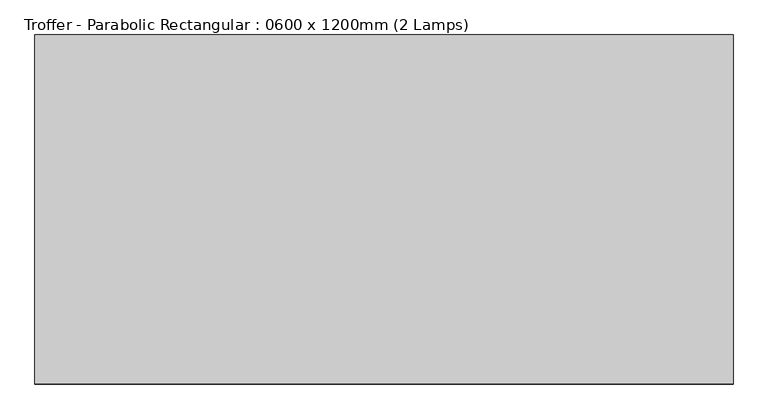
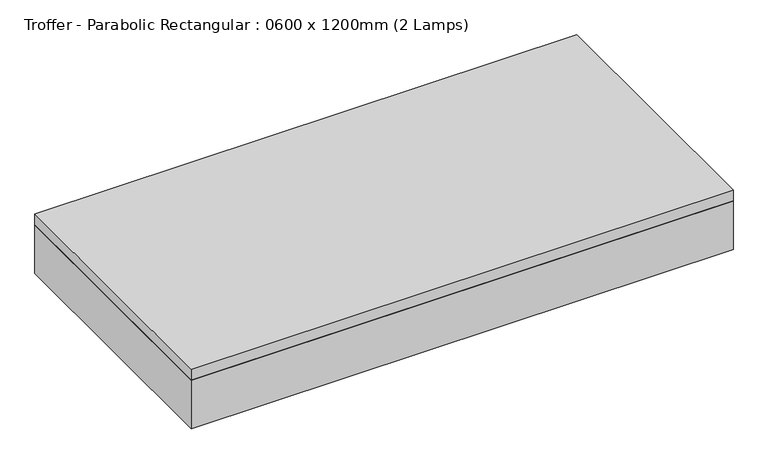
"""IFC4 building model written with IfcOpenShell, lengths in millimetres: light fixture geometry, Troffer - Parabolic Rectangular : 0600 x 1200mm (2 Lamps)."""

from ifc_helpers import new_model, si_unit, frame, origin, place, context, project, spatial, polyline, outline, extrude, source, transform, mapped, element, save


def troffer_parabolic_rectangular_0600_x_1200mm_2_lamps_e156559b(model_context):
    return source(origin(), model_context, "Body", "SweptSolid", [
        extrude(outline(polyline([(565.4964984, 219.9340679), (565.4964984, -338.8659321), (-602.9035016, -338.8659321), (-602.9035016, 219.9340679), (565.4964984, 219.9340679)]), holes=[polyline([(-409.2285016, 35.7840679), (-409.2285016, 213.5840679), (-596.5535016, 213.5840679), (-596.5535016, 35.7840679), (-409.2285016, 35.7840679)]), polyline([(-409.2285016, -148.3659321), (-409.2285016, 29.4340679), (-596.5535016, 29.4340679), (-596.5535016, -148.3659321), (-409.2285016, -148.3659321)]), polyline([(-409.2285016, -154.7159321), (-596.5535016, -154.7159321), (-596.5535016, -332.5159321), (-409.2285016, -332.5159321), (-409.2285016, -154.7159321)]), polyline([(-215.5535016, 35.7840679), (-215.5535016, 213.5840679), (-402.8785016, 213.5840679), (-402.8785016, 35.7840679), (-215.5535016, 35.7840679)]), polyline([(-215.5535016, -148.3659321), (-215.5535016, 29.4340679), (-402.8785016, 29.4340679), (-402.8785016, -148.3659321), (-215.5535016, -148.3659321)]), polyline([(-215.5535016, -154.7159321), (-402.8785016, -154.7159321), (-402.8785016, -332.5159321), (-215.5535016, -332.5159321), (-215.5535016, -154.7159321)]), polyline([(-21.8785016, 35.7840679), (-21.8785016, 213.5840679), (-209.2035016, 213.5840679), (-209.2035016, 35.7840679), (-21.8785016, 35.7840679)]), polyline([(-21.8785016, -148.3659321), (-21.8785016, 29.4340679), (-209.2035016, 29.4340679), (-209.2035016, -148.3659321), (-21.8785016, -148.3659321)]), polyline([(-21.8785016, -154.7159321), (-209.2035016, -154.7159321), (-209.2035016, -332.5159321), (-21.8785016, -332.5159321), (-21.8785016, -154.7159321)]), polyline([(171.7964984, 35.7840679), (171.7964984, 213.5840679), (-15.5285016, 213.5840679), (-15.5285016, 35.7840679), (171.7964984, 35.7840679)]), polyline([(171.7964984, -148.3659321), (171.7964984, 29.4340679), (-15.5285016, 29.4340679), (-15.5285016, -148.3659321), (171.7964984, -148.3659321)]), polyline([(171.7964984, -154.7159321), (-15.5285016, -154.7159321), (-15.5285016, -332.5159321), (171.7964984, -332.5159321), (171.7964984, -154.7159321)]), polyline([(365.4714984, 35.7840679), (365.4714984, 213.5840679), (178.1464984, 213.5840679), (178.1464984, 35.7840679), (365.4714984, 35.7840679)]), polyline([(365.4714984, -148.3659321), (365.4714984, 29.4340679), (178.1464984, 29.4340679), (178.1464984, -148.3659321), (365.4714984, -148.3659321)]), polyline([(365.4714984, -154.7159321), (178.1464984, -154.7159321), (178.1464984, -332.5159321), (365.4714984, -332.5159321), (365.4714984, -154.7159321)]), polyline([(559.1464984, 35.7840679), (559.1464984, 213.5840679), (371.8214984, 213.5840679), (371.8214984, 35.7840679), (559.1464984, 35.7840679)]), polyline([(559.1464984, -148.3659321), (559.1464984, 29.4340679), (371.8214984, 29.4340679), (371.8214984, -148.3659321), (559.1464984, -148.3659321)]), polyline([(559.1464984, -154.7159321), (371.8214984, -154.7159321), (371.8214984, -332.5159321), (559.1464984, -332.5159321), (559.1464984, -154.7159321)])]), frame((0.0, 0.0, 2438.4), z_axis=(0.0, 0.0, 1.0), x_axis=(1.0, 0.0, 0.0)), (0.0, 0.0, 1.0), 3.175),
        extrude(outline(polyline([(555.8964984, 215.1340679), (555.8964984, -334.0659321), (-593.3035016, -334.0659321), (-593.3035016, 215.1340679), (555.8964984, 215.1340679)])), frame((0.0, 0.0, 2514.6), z_axis=(0.0, 0.0, 1.0), x_axis=(1.0, 0.0, 0.0)), (0.0, 0.0, 1.0), 6.35),
        extrude(outline(polyline([(565.4964984, 219.9340679), (565.4964984, -338.8659321), (-602.9035016, -338.8659321), (-602.9035016, 219.9340679), (565.4964984, 219.9340679)]), holes=[polyline([(-409.2285016, 35.7840679), (-409.2285016, 213.5840679), (-596.5535016, 213.5840679), (-596.5535016, 35.7840679), (-409.2285016, 35.7840679)]), polyline([(-409.2285016, -148.3659321), (-409.2285016, 29.4340679), (-596.5535016, 29.4340679), (-596.5535016, -148.3659321), (-409.2285016, -148.3659321)]), polyline([(-409.2285016, -154.7159321), (-596.5535016, -154.7159321), (-596.5535016, -332.5159321), (-409.2285016, -332.5159321), (-409.2285016, -154.7159321)]), polyline([(-215.5535016, 35.7840679), (-215.5535016, 213.5840679), (-402.8785016, 213.5840679), (-402.8785016, 35.7840679), (-215.5535016, 35.7840679)]), polyline([(-215.5535016, -148.3659321), (-215.5535016, 29.4340679), (-402.8785016, 29.4340679), (-402.8785016, -148.3659321), (-215.5535016, -148.3659321)]), polyline([(-215.5535016, -154.7159321), (-402.8785016, -154.7159321), (-402.8785016, -332.5159321), (-215.5535016, -332.5159321), (-215.5535016, -154.7159321)]), polyline([(-21.8785016, 35.7840679), (-21.8785016, 213.5840679), (-209.2035016, 213.5840679), (-209.2035016, 35.7840679), (-21.8785016, 35.7840679)]), polyline([(-21.8785016, -148.3659321), (-21.8785016, 29.4340679), (-209.2035016, 29.4340679), (-209.2035016, -148.3659321), (-21.8785016, -148.3659321)]), polyline([(-21.8785016, -154.7159321), (-209.2035016, -154.7159321), (-209.2035016, -332.5159321), (-21.8785016, -332.5159321), (-21.8785016, -154.7159321)]), polyline([(171.7964984, 35.7840679), (171.7964984, 213.5840679), (-15.5285016, 213.5840679), (-15.5285016, 35.7840679), (171.7964984, 35.7840679)]), polyline([(171.7964984, -148.3659321), (171.7964984, 29.4340679), (-15.5285016, 29.4340679), (-15.5285016, -148.3659321), (171.7964984, -148.3659321)]), polyline([(171.7964984, -154.7159321), (-15.5285016, -154.7159321), (-15.5285016, -332.5159321), (171.7964984, -332.5159321), (171.7964984, -154.7159321)]), polyline([(365.4714984, 35.7840679), (365.4714984, 213.5840679), (178.1464984, 213.5840679), (178.1464984, 35.7840679), (365.4714984, 35.7840679)]), polyline([(365.4714984, -148.3659321), (365.4714984, 29.4340679), (178.1464984, 29.4340679), (178.1464984, -148.3659321), (365.4714984, -148.3659321)]), polyline([(365.4714984, -154.7159321), (178.1464984, -154.7159321), (178.1464984, -332.5159321), (365.4714984, -332.5159321), (365.4714984, -154.7159321)]), polyline([(559.1464984, 35.7840679), (559.1464984, 213.5840679), (371.8214984, 213.5840679), (371.8214984, 35.7840679), (559.1464984, 35.7840679)]), polyline([(559.1464984, -148.3659321), (559.1464984, 29.4340679), (371.8214984, 29.4340679), (371.8214984, -148.3659321), (559.1464984, -148.3659321)]), polyline([(559.1464984, -154.7159321), (371.8214984, -154.7159321), (371.8214984, -332.5159321), (559.1464984, -332.5159321), (559.1464984, -154.7159321)])]), frame((0.0, 0.0, 2441.575), z_axis=(0.0, 0.0, 1.0), x_axis=(1.0, 0.0, 0.0)), (0.0, 0.0, 1.0), 47.625),
        extrude(outline(polyline([(581.2964984, 240.5340679), (581.2964984, -359.4659321), (-618.7035016, -359.4659321), (-618.7035016, 240.5340679), (581.2964984, 240.5340679)]), holes=[polyline([(555.8964984, 215.1340679), (-593.3035016, 215.1340679), (-593.3035016, -334.0659321), (555.8964984, -334.0659321), (555.8964984, 215.1340679)])]), frame((0.0, 0.0, 2438.4), z_axis=(0.0, 0.0, 1.0), x_axis=(1.0, 0.0, 0.0)), (0.0, 0.0, 1.0), 114.3),
        extrude(outline(polyline([(581.2964984, 240.5340679), (581.2964984, -359.4659321), (-618.7035016, -359.4659321), (-618.7035016, 240.5340679), (581.2964984, 240.5340679)])), frame((0.0, 0.0, 2552.7), z_axis=(0.0, 0.0, 1.0), x_axis=(1.0, 0.0, 0.0)), (0.0, 0.0, 1.0), 25.4),
    ])


if __name__ == "__main__":
    model = new_model("IFC4")
    model_context = context("Model", 3, world=origin())
    ifc_project = project(units=[si_unit("LENGTHUNIT", "METRE", prefix="MILLI")], contexts=[model_context])
    site = spatial("IfcSite", under=ifc_project)
    building = spatial("IfcBuilding", under=site)
    placement = place(None, origin())
    troffer_parabolic_rectangular_0600_x_1200mm_2_lamps_shape = troffer_parabolic_rectangular_0600_x_1200mm_2_lamps_e156559b(model_context)
    element("IfcLightFixture", 1, ObjectType="Troffer - Parabolic Rectangular : 0600 x 1200mm (2 Lamps)", at=placement, inside=building, context=model_context, shape_type="MappedRepresentation", body=[
        mapped(troffer_parabolic_rectangular_0600_x_1200mm_2_lamps_shape, transform((0.0, 0.0, 0.0), x_axis=(1.0, 0.0, 0.0), y_axis=(0.0, 1.0, 0.0), z_axis=(0.0, 0.0, 1.0))),
    ])
    save(model, "model.ifc")

# Revit data of these elements
# Type "Troffer - Parabolic Rectangular : 0600 x 1200mm (2 Lamps)"
#   Lamp = "T-12"
#   Wattage Comments = "(2)20"
#   Wattage = 80 W
#   built-in parameter 1150110 = 1 (stored number, unit not read)
#   built-in parameter 1114217 = 1 (stored number, unit not read)
#   built-in parameter 1150109 = 1 (stored number, unit not read)
#   built-in parameter 1150113 = 1 (stored number, unit not read)
#   built-in parameter 1150105 = 2037.18 (stored number, unit not read)
#   built-in parameter 1150115 = 1 (stored number, unit not read)
#   Light Source Symbol Size = 609.6 mm
#   built-in parameter 1150112 = 1 (stored number, unit not read)
#   built-in parameter 1150114 = 1 (stored number, unit not read)
#   built-in parameter 1150107 = 4230 (stored number, unit not read)
#   built-in parameter 1150106 = 20.3718 (stored number, unit not read)
#   Emit from Rectangle Width = 550 mm
#   Emit from Rectangle Length = 1150 mm
#   built-in parameter 1150104 = 7.43224 (stored number, unit not read)
#   Circle Width = 360 mm
#   Lumens = 6400 lm
#   built-in parameter 1114218 = 1 (stored number, unit not read)
#   built-in parameter 1150133 = 10 (stored number, unit not read)
#   built-in parameter 1150134 = 8
#   Color Filter = 16777215
#   Diffuser = Metal - Chrome
#   Light Box = Metal - Chrome
#   Emit Shape Visible in Rendering = no
#   Dimming Lamp Color Temperature Shift = (empty or 0)
#   Default Elevation = 0
# Element 1 (IfcLightFixture, "Troffer - Parabolic Rectangular : 0600 x 1200mm (2 Lamps)")
#   Materials on its faces: "Metal - Chrome"
# Materials
#   "Metal - Chrome": class "Metal", colour RGB 247 247 247, transparency 0
